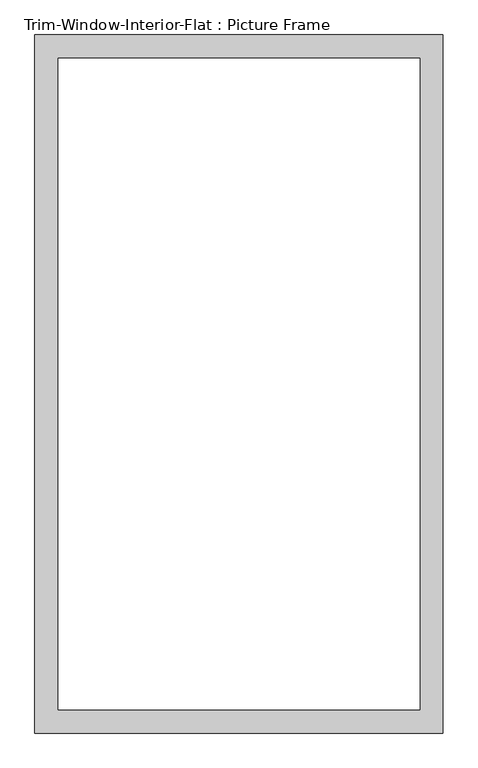
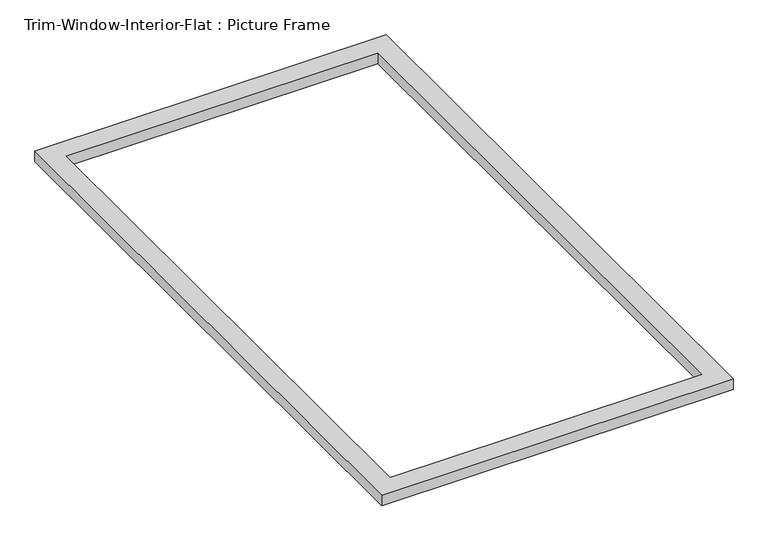
"""IFC4 building model written with IfcOpenShell, lengths in millimetres: proxy geometry, Trim-Window-Interior-Flat : Picture Frame."""

from ifc_helpers import new_model, si_unit, origin, origin_with_axes, place, context, project, spatial, polyline, outline, extrude, source, transform, mapped, element, save


def trim_window_interior_flat_picture_frame_cf830d55(model_context):
    return source(origin(), model_context, "Body", "SweptSolid", [
        extrude(outline(polyline([(501.65, -44.45), (-501.65, -44.45), (-501.65, 1670.05), (501.65, 1670.05), (501.65, -44.45)]), holes=[polyline([(444.5, 12.7), (444.5, 1612.9), (-444.5, 1612.9), (-444.5, 12.7), (444.5, 12.7)])]), origin_with_axes(), (0.0, 0.0, 1.0), 31.75),
    ])


if __name__ == "__main__":
    model = new_model("IFC4")
    model_context = context("Model", 3, world=origin())
    ifc_project = project(units=[si_unit("LENGTHUNIT", "METRE", prefix="MILLI")], contexts=[model_context])
    site = spatial("IfcSite", under=ifc_project)
    building = spatial("IfcBuilding", under=site)
    placement = place(None, origin())
    trim_window_interior_flat_picture_frame_shape = trim_window_interior_flat_picture_frame_cf830d55(model_context)
    element("IfcBuildingElementProxy", 1, Name="Trim-Window-Interior-Flat : Picture Frame", ObjectType="Trim-Window-Interior-Flat : Picture Frame", at=placement, inside=building, context=model_context, shape_type="MappedRepresentation", body=[
        mapped(trim_window_interior_flat_picture_frame_shape, transform((0.0, 0.0, 0.0), x_axis=(1.0, 0.0, 0.0), y_axis=(0.0, 1.0, 0.0), z_axis=(0.0, 0.0, 1.0))),
    ])
    save(model, "model.ifc")

# Revit data of these elements
# Type "Trim-Window-Interior-Flat : Picture Frame"
#   Trim Thickness_Picture Frame = 0' - 1 1/4"
#   Trim Width = 0' - 2 1/4"
#   Trim Thickness_with Sill = 0' - 0 3/4"
#   Sill Thickness = 0' - 1 1/4"
#   Opening Width [instance default] = 2' - 0"
#   Opening Height [instance default] = 3' - 0"
#   Default Elevation = 4' - 0"
#   Sill = no
#   Picture Frame = yes
#   Trim Material [instance default] = none
# Element 1 (IfcBuildingElementProxy, "Trim-Window-Interior-Flat : Picture Frame")
#   Opening Width = 3' - 0"
#   Opening Height = 5' - 4"
#   Trim Material = Wood - Stained
#   Materials on its faces: "Wood - Stained"
# Materials
#   "Wood - Stained": class "Wood", colour RGB 224 178 126, transparency 0, Cost = 0
